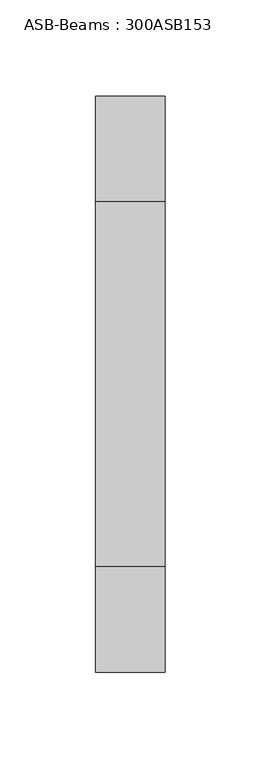
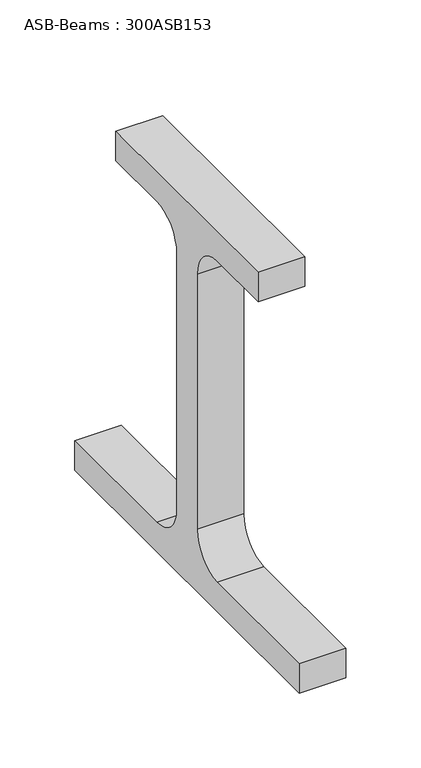
"""IFC4 building model written with IfcOpenShell, lengths in millimetres: beam geometry, ASB-Beams : 300ASB153."""

from ifc_helpers import new_model, si_unit, point, frame, frame_2d, origin, place, context, project, spatial, polyline, circle_curve, trimmed, segment, composite_curve, outline, extrude, source, transform, mapped, element, save


def asb_beams_300asb153_cd404b0f(model_context):
    return source(origin(), model_context, "Body", "SweptSolid", [
        extrude(outline(composite_curve([segment(polyline([(95.0, 174.0), (95.0, 150.0), (40.5, 150.0)]), True, "CONTINUOUS"), segment(trimmed(circle_curve(frame_2d((40.5, 123.0)), 27.0), [point((40.5, 150.0))], [point((13.5, 123.0))], True, "CARTESIAN"), True, "CONTINUOUS"), segment(polyline([(13.5, 123.0), (13.5, -85.0)]), True, "CONTINUOUS"), segment(trimmed(circle_curve(frame_2d((40.5, -85.0)), 27.0), [point((13.5, -85.0))], [point((40.5, -112.0))], True, "CARTESIAN"), True, "CONTINUOUS"), segment(polyline([(40.5, -112.0), (150.0, -112.0), (150.0, -136.0), (-150.0, -136.0), (-150.0, -112.0), (-40.5, -112.0)]), True, "CONTINUOUS"), segment(trimmed(circle_curve(frame_2d((-40.5, -85.0)), 27.0), [point((-40.5, -112.0))], [point((-13.5, -85.0))], True, "CARTESIAN"), True, "CONTINUOUS"), segment(polyline([(-13.5, -85.0), (-13.5, 123.0)]), True, "CONTINUOUS"), segment(trimmed(circle_curve(frame_2d((-40.5, 123.0)), 27.0), [point((-13.5, 123.0))], [point((-40.5, 150.0))], True, "CARTESIAN"), True, "CONTINUOUS"), segment(polyline([(-40.5, 150.0), (-95.0, 150.0), (-95.0, 174.0), (95.0, 174.0)]), True, "CONTINUOUS")], self_intersect=False)), frame((-176.5, 0.0, 0.0), z_axis=(1.0, 0.0, 0.0), x_axis=(0.0, 1.0, 0.0)), (0.0, 0.0, 1.0), 36.0),
    ])


if __name__ == "__main__":
    model = new_model("IFC4")
    model_context = context("Model", 3, world=origin())
    ifc_project = project(units=[si_unit("LENGTHUNIT", "METRE", prefix="MILLI")], contexts=[model_context])
    site = spatial("IfcSite", under=ifc_project)
    building = spatial("IfcBuilding", under=site)
    placement = place(None, origin())
    asb_beams_300asb153_shape = asb_beams_300asb153_cd404b0f(model_context)
    element("IfcBeam", 1, ObjectType="ASB-Beams : 300ASB153", at=placement, inside=building, context=model_context, shape_type="MappedRepresentation", body=[
        mapped(asb_beams_300asb153_shape, transform((0.0, 0.0, 0.0), x_axis=(1.0, 0.0, 0.0), y_axis=(0.0, 1.0, 0.0), z_axis=(0.0, 0.0, 1.0))),
    ])
    save(model, "model.ifc")

# Revit data of these elements
# Type "ASB-Beams : 300ASB153"
#   Description = "305 x 305 RSJ"
#   Type Comments = "Steel 50-355"
#   ye = 174 mm
#   t = 27 mm
#   r = 27 mm
#   k = 51 mm
#   W = 0.1528
#   T = 24 mm
#   Start Extension Calculation [instance default] = 3000 mm
#   Start Extension [instance default] = -12.7 mm
#   End Extension Calculation [instance default] = 3000 mm
#   End Extension [instance default] = -12.7 mm
#   D = 310 mm
#   Bt = 190 mm
#   Bb = 300 mm
#   Length [instance default] = 1500 mm
#   A = 0.0195 m²
#   Structural Material [instance default] = Metal - Steel 50-355
#   Assembly Code = ""
# Element 1 (IfcBeam, "ASB-Beams : 300ASB153")
#   Materials on its faces: "Metal - Steel 50-355"
# Materials
#   "Metal - Steel 50-355": class "Metal", colour RGB 247 247 247, transparency 0
